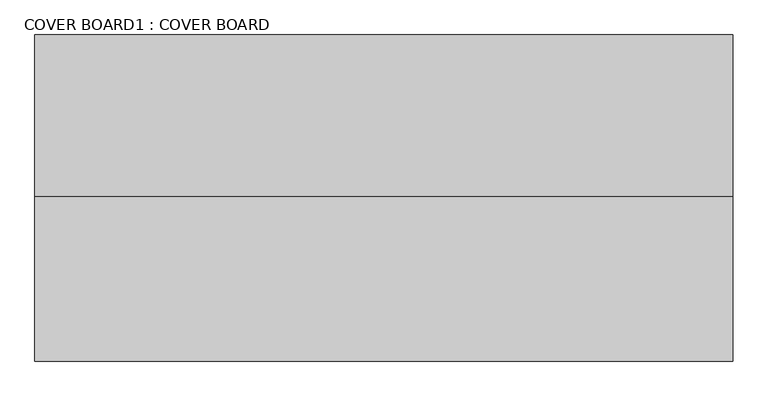
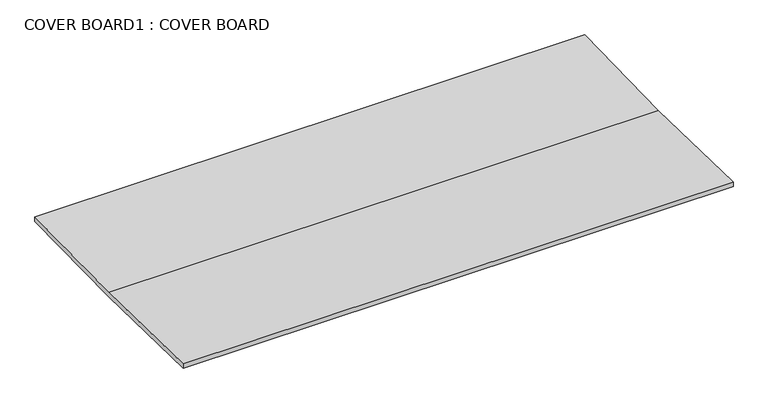
"""IFC4 building model written with IfcOpenShell, lengths in millimetres: proxy geometry, COVER BOARD1 : COVER BOARD."""

import ifcopenshell
import ifcopenshell.guid

model = None  # the IFC model being written
_history = None  # IfcOwnerHistory: only IFC2X3 demands one
_inside = {}  # id of a spatial element -> (the spatial element, [elements in it])
_under = {}  # id of a project, library or spatial element -> (it, [spatial elements below it])
_declared = {}  # id of a project -> (the project, [libraries it declares])
_typed = {}  # id of a type object -> (the type object, [elements of that type])
_made_of = {}  # id of a material, layer set ... -> (it, [elements and type objects made of it])


def new_model(schema):
    """Start an empty IFC model of exactly this schema.

    Asked for "IFC4X3", IfcOpenShell would pick the latest addendum, in which some entities
    have other attributes; the version numbers below select the first issue.
    IFC2X3 requires an IfcOwnerHistory on every rooted entity: one is made here for all.
    """
    global model, _history
    if schema == "IFC4X3":
        model = ifcopenshell.file(schema_version=(4, 3, 0, 0))
    else:
        model = ifcopenshell.file(schema=schema)
    _inside.clear()
    _under.clear()
    _declared.clear()
    _typed.clear()
    _made_of.clear()
    _history = None
    if model.schema == "IFC2X3":
        org = make("IfcOrganization", Name="unknown")
        user = make(
            "IfcPersonAndOrganization",
            ThePerson=make("IfcPerson", FamilyName="unknown"),
            TheOrganization=org,
        )
        app = make(
            "IfcApplication",
            ApplicationDeveloper=org,
            Version="unknown",
            ApplicationFullName="unknown",
            ApplicationIdentifier="unknown",
        )
        _history = make(
            "IfcOwnerHistory",
            OwningUser=user,
            OwningApplication=app,
            ChangeAction="ADDED",
            CreationDate=0,
        )
    return model


def make(cls, **values):
    """One entity of the class cls with the attributes given. An attribute that is None is left unset."""
    return model.create_entity(
        cls, **{name: value for name, value in values.items() if value is not None}
    )


def rooted(cls, **values):
    """An entity with a GlobalId (a new one), such as an element, a storey or a relation."""
    return make(cls, GlobalId=ifcopenshell.guid.new(), OwnerHistory=_history, **values)


def si_unit(unit_type, name, prefix=None):
    """IfcSIUnit, for example si_unit("LENGTHUNIT", "METRE", prefix="MILLI")."""
    return make("IfcSIUnit", UnitType=unit_type, Prefix=prefix, Name=name)


def assignment(units):
    """IfcUnitAssignment: the units of a project."""
    return None if units is None else make("IfcUnitAssignment", Units=units)


def point(xyz):
    """IfcCartesianPoint."""
    return None if xyz is None else make("IfcCartesianPoint", Coordinates=xyz)


def direction(xyz):
    """IfcDirection."""
    return None if xyz is None else make("IfcDirection", DirectionRatios=xyz)


def frame(location, z_axis=None, x_axis=None):
    """IfcAxis2Placement3D, a coordinate frame: its origin and axes. An axis left out is left unset."""
    return make(
        "IfcAxis2Placement3D",
        Location=point(location),
        Axis=direction(z_axis),
        RefDirection=direction(x_axis),
    )


def origin():
    """The frame at (0, 0, 0) with its axes left unset."""
    return frame((0.0, 0.0, 0.0))


def place(relative_to, where):
    """IfcLocalPlacement: puts the frame where relative to a parent placement (None: the world)."""
    return make(
        "IfcLocalPlacement", PlacementRelTo=relative_to, RelativePlacement=where
    )


def context(
    kind, dimensions, precision=None, world=None, true_north=None, identifier=None
):
    """IfcGeometricRepresentationContext, for example the 3D "Model" context."""
    return make(
        "IfcGeometricRepresentationContext",
        ContextIdentifier=identifier,
        ContextType=kind,
        CoordinateSpaceDimension=dimensions,
        Precision=precision,
        WorldCoordinateSystem=world,
        TrueNorth=true_north,
    )


def project(units=None, contexts=None):
    """IfcProject with its units and contexts."""
    return rooted(
        "IfcProject",
        Name="project",
        RepresentationContexts=contexts,
        UnitsInContext=assignment(units),
    )


def spatial(cls, under=None, at=None, **own):
    """A site, building, storey or space (cls), placed at a placement, below another one or the project."""
    s = rooted(cls, ObjectPlacement=at, **own)
    if under is not None:
        _under.setdefault(under.id(), (under, []))[1].append(s)
    return s


def polyline(points):
    """IfcPolyline through the points."""
    return make("IfcPolyline", Points=[point(p) for p in points])


def outline(outer, holes=None, kind="AREA"):
    """IfcArbitraryClosedProfileDef: a profile drawn as a closed curve; with holes, ...WithVoids."""
    if holes is None:
        return make("IfcArbitraryClosedProfileDef", ProfileType=kind, OuterCurve=outer)
    return make(
        "IfcArbitraryProfileDefWithVoids",
        ProfileType=kind,
        OuterCurve=outer,
        InnerCurves=holes,
    )


def extrude(swept, where, along, depth):
    """IfcExtrudedAreaSolid: the profile swept, set in the frame where, extruded along a direction by depth."""
    return make(
        "IfcExtrudedAreaSolid",
        SweptArea=swept,
        Position=where,
        ExtrudedDirection=direction(along),
        Depth=depth,
    )


def shape(context_of_items, identifier, shape_type, items):
    """IfcShapeRepresentation: the items that make up one representation, for example the "Body"."""
    return make(
        "IfcShapeRepresentation",
        ContextOfItems=context_of_items,
        RepresentationIdentifier=identifier,
        RepresentationType=shape_type,
        Items=items,
    )


def source(mapping_origin, context_of_items, identifier, shape_type, items):
    """IfcRepresentationMap: a shape defined once, which mapped items show again and again."""
    return make(
        "IfcRepresentationMap",
        MappingOrigin=mapping_origin,
        MappedRepresentation=shape(context_of_items, identifier, shape_type, items),
    )


def transform(
    local_origin,
    x_axis=None,
    y_axis=None,
    z_axis=None,
    scale=None,
    scale2=None,
    scale3=None,
    uniform=True,
):
    """IfcCartesianTransformationOperator3D, or its non-uniform kind. x_axis, y_axis, z_axis: its Axis1, 2, 3."""
    if uniform:
        return make(
            "IfcCartesianTransformationOperator3D",
            Axis1=direction(x_axis),
            Axis2=direction(y_axis),
            LocalOrigin=point(local_origin),
            Scale=scale,
            Axis3=direction(z_axis),
        )
    return make(
        "IfcCartesianTransformationOperator3DnonUniform",
        Axis1=direction(x_axis),
        Axis2=direction(y_axis),
        LocalOrigin=point(local_origin),
        Scale=scale,
        Axis3=direction(z_axis),
        Scale2=scale2,
        Scale3=scale3,
    )


def mapped(mapping_source, mapping_target):
    """IfcMappedItem: shows the shape of a source again, moved by a transform."""
    return make(
        "IfcMappedItem", MappingSource=mapping_source, MappingTarget=mapping_target
    )


def made_of(thing, what):
    """Note that an element or type object is made of a material, layer set ...; save() writes the relation."""
    if what is not None:
        _made_of.setdefault(what.id(), (what, []))[1].append(thing)
    return thing


def element(
    cls,
    number,
    at=None,
    inside=None,
    cuts=None,
    type_object=None,
    material=None,
    context=None,
    identifier="Body",
    shape_type=None,
    held_by="IfcProductDefinitionShape",
    body=None,
    shapes=None,
    **own,
):
    """One element of the class cls, such as IfcWall. Its Tag is "e" and its number.

    at: its placement. inside: the storey or other place that contains it. cuts: it is an
    opening in that element (IfcRelVoidsElement). A single representation is given by context,
    identifier, shape_type and body (its items); several are given by shapes. held_by: the class
    of the entity that holds the representations. save() writes the other relations.
    """
    e = rooted(cls, Tag="e%d" % number, ObjectPlacement=at, **own)
    if body is not None:
        shapes = [shape(context, identifier, shape_type, body)]
    if shapes is not None:
        e.Representation = make(held_by, Representations=shapes)
    if inside is not None:
        _inside.setdefault(inside.id(), (inside, []))[1].append(e)
    if cuts is not None:
        rooted(
            "IfcRelVoidsElement", RelatingBuildingElement=cuts, RelatedOpeningElement=e
        )
    if type_object is not None:
        _typed.setdefault(type_object.id(), (type_object, []))[1].append(e)
    return made_of(e, material)


def aggregate(whole, parts):
    """IfcRelAggregates: a whole, such as a stair, and the parts it consists of."""
    return rooted("IfcRelAggregates", RelatingObject=whole, RelatedObjects=parts)


def save(model, path):
    """Write the relations noted so far, then the file.

    IfcRelAggregates (storeys below a building ...), IfcRelContainedInSpatialStructure (elements
    in a storey), IfcRelDefinesByType, IfcRelAssociatesMaterial and IfcRelDeclares: one each for
    every whole, place, type object, material and project.
    """
    for whole, parts in _under.values():
        aggregate(whole, parts)
    for where, things in _inside.values():
        rooted(
            "IfcRelContainedInSpatialStructure",
            RelatedElements=things,
            RelatingStructure=where,
        )
    for kind, things in _typed.values():
        rooted("IfcRelDefinesByType", RelatedObjects=things, RelatingType=kind)
    for what, things in _made_of.values():
        rooted("IfcRelAssociatesMaterial", RelatedObjects=things, RelatingMaterial=what)
    for by, libraries in _declared.values():
        rooted("IfcRelDeclares", RelatingContext=by, RelatedDefinitions=libraries)
    model.write(path)


def cover_board1_cover_board_90439fdb(model_context):
    return source(origin(), model_context, "Body", "SweptSolid", [
        extrude(outline(polyline([(-4872.9612169, 40211.218553), (-4408.9401513, 40221.0164062), (-4408.9401513, 40203.6846871), (-4872.9612169, 40193.8868338), (-5343.2581759, 40203.6846871), (-5343.2581759, 40221.0164063), (-4872.9612169, 40211.218553)])), frame((12382.7678845, 0.0, 0.0), z_axis=(1.0, 0.0, 0.0), x_axis=(0.0, 1.0, 0.0)), (0.0, 0.0, 1.0), 2000.0),
    ])


if __name__ == "__main__":
    model = new_model("IFC4")
    model_context = context("Model", 3, world=origin())
    ifc_project = project(units=[si_unit("LENGTHUNIT", "METRE", prefix="MILLI")], contexts=[model_context])
    site = spatial("IfcSite", under=ifc_project)
    building = spatial("IfcBuilding", under=site)
    placement = place(None, origin())
    cover_board1_cover_board_shape = cover_board1_cover_board_90439fdb(model_context)
    element("IfcBuildingElementProxy", 1, Name="COVER BOARD1 : COVER BOARD", ObjectType="COVER BOARD1 : COVER BOARD", at=placement, inside=building, context=model_context, shape_type="MappedRepresentation", body=[
        mapped(cover_board1_cover_board_shape, transform((0.0, 0.0, 0.0), x_axis=(1.0, 0.0, 0.0), y_axis=(0.0, 1.0, 0.0), z_axis=(0.0, 0.0, 1.0))),
    ])
    save(model, "model.ifc")

# Revit data of these elements
# Type "COVER BOARD1 : COVER BOARD"
#   NameOverride = "COVER BOARD"
# Element 1 (IfcBuildingElementProxy, "COVER BOARD1 : COVER BOARD")
#   Materials on its faces: "CDX PLYWOOD - SEE STRUCTURAL DWGS"
# Materials
#   "CDX PLYWOOD - SEE STRUCTURAL DWGS": class "Unassigned", colour RGB 202 163 108, transparency 0, Cost = 0
